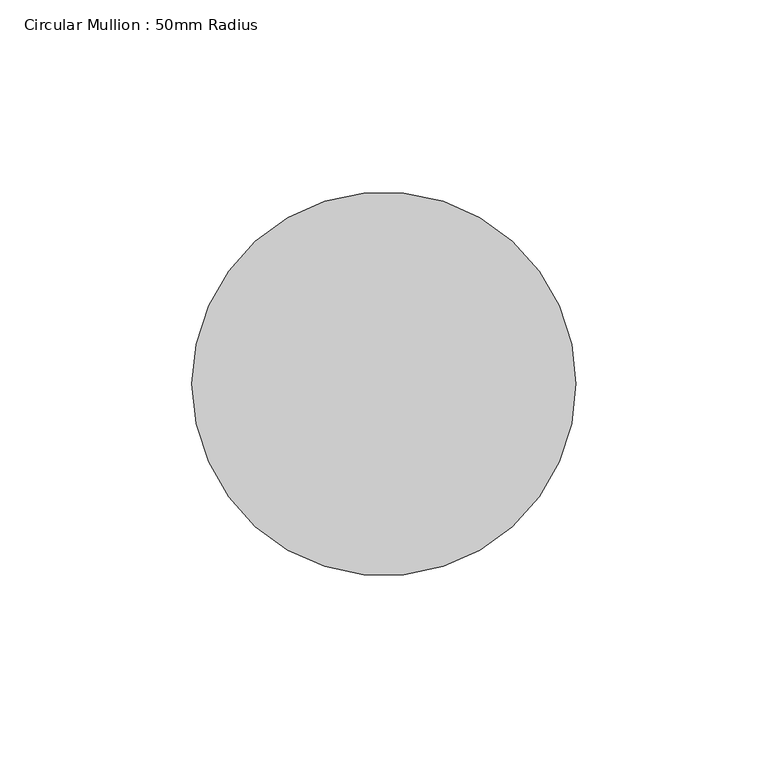
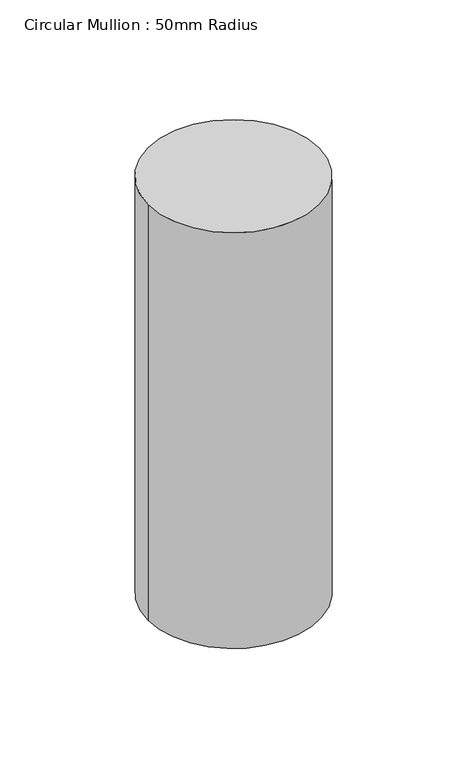
"""IFC4 building model written with IfcOpenShell, lengths in millimetres: member geometry, Circular Mullion : 50mm Radius."""

from ifc_helpers import new_model, si_unit, point, frame, origin, origin_2d, place, context, project, spatial, circle_curve, trimmed, segment, composite_curve, outline, extrude, source, transform, mapped, element, save


def circular_mullion_50mm_radius_13f31984(model_context):
    return source(origin(), model_context, "Body", "SweptSolid", [
        extrude(outline(composite_curve([segment(trimmed(circle_curve(origin_2d(), 50.0), [point((50.0, 0.0))], [point((-50.0, 0.0))], False, "CARTESIAN"), True, "CONTINUOUS"), segment(trimmed(circle_curve(origin_2d(), 50.0), [point((-50.0, 0.0))], [point((50.0, 0.0))], False, "CARTESIAN"), True, "CONTINUOUS")], self_intersect=False)), frame((0.0, 0.0, -256.8752499), z_axis=(0.0, 0.0, 1.0), x_axis=(1.0, 0.0, 0.0)), (0.0, 0.0, 1.0), 256.8752499),
    ])


if __name__ == "__main__":
    model = new_model("IFC4")
    model_context = context("Model", 3, world=origin())
    ifc_project = project(units=[si_unit("LENGTHUNIT", "METRE", prefix="MILLI")], contexts=[model_context])
    site = spatial("IfcSite", under=ifc_project)
    building = spatial("IfcBuilding", under=site)
    placement = place(None, origin())
    circular_mullion_50mm_radius_shape = circular_mullion_50mm_radius_13f31984(model_context)
    element("IfcMember", 1, ObjectType="Circular Mullion : 50mm Radius", at=placement, inside=building, context=model_context, shape_type="MappedRepresentation", body=[
        mapped(circular_mullion_50mm_radius_shape, transform((0.0, 0.0, 0.0), x_axis=(1.0, 0.0, 0.0), y_axis=(0.0, 1.0, 0.0), z_axis=(0.0, 0.0, 1.0))),
    ])
    save(model, "model.ifc")

# Revit data of these elements
# Type "Circular Mullion : 50mm Radius"
#   built-in parameter 1007350 = 0.164042 (stored number, unit not read)
# Element 1 (IfcMember, "Circular Mullion : 50mm Radius")
#   Materials on its faces: "Aluminium"
# Materials
#   "Aluminium": class "Metal", colour RGB 247 247 247, transparency 0, Description = "Aluminium 6061", Cost = 0
